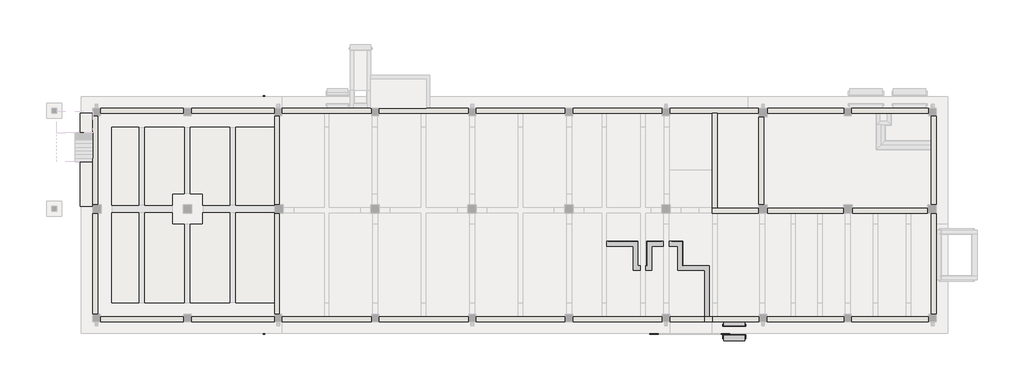
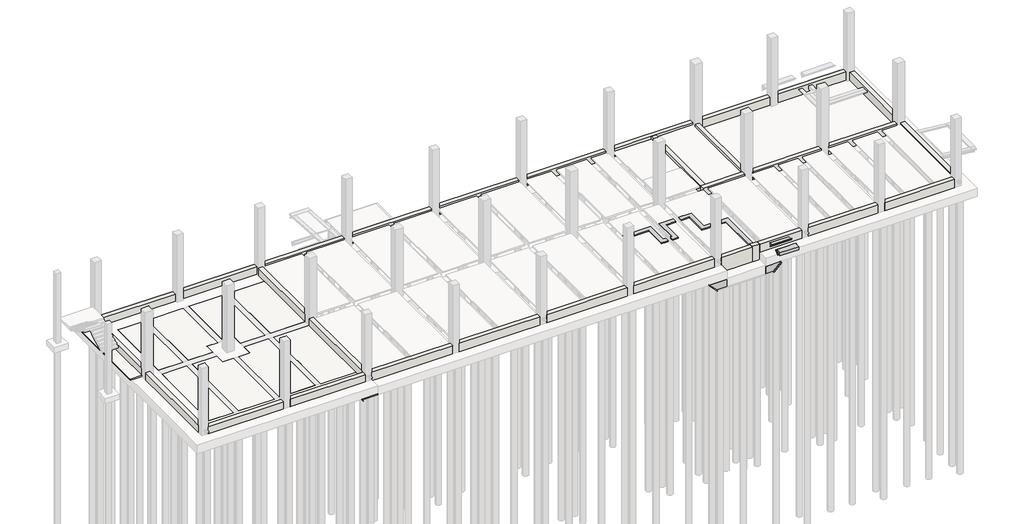
# One storey, part 1 of 7: 31 walls, 12 proxies, 4 slabs.
"""IFC4 building model written with IfcOpenShell, lengths in millimetres."""

from ifc_helpers import new_model, si_unit, frame, origin, place, context, project, spatial, polyline, outline, extrude, faceted_brep, element, save

model = new_model("IFC4")

# Units and contexts
model_context = context("Model", 3, world=origin())
ifc_project = project(units=[si_unit("LENGTHUNIT", "METRE", prefix="MILLI")], contexts=[model_context])

# Site, building, storey
site = spatial("IfcSite", under=ifc_project)
building = spatial("IfcBuilding", under=site)
storey = spatial("IfcBuildingStorey", under=building, Name="H.P.P", Elevation=4500.0)

# Proxies
placement = place(None, origin())
element("IfcBuildingElementProxy", 1, Name="H_SF_AR_S17_SOG Edge_1625x700", ObjectType="H_SF_AR_S17_SOG Edge_1625x700", at=placement, inside=storey, context=model_context, shape_type="SweptSolid", body=[
    extrude(outline(polyline([(2500.0, 47300.0), (3200.0, 47300.0), (3200.0, 45675.0), (2500.0, 46375.0), (2500.0, 47300.0)])), frame((0.0, -18250.0000001, 0.0), z_axis=(0.0, 1.0, 0.0), x_axis=(0.0, 0.0, 1.0)), (0.0, 0.0, 1.0), 2500.0),
])
element("IfcBuildingElementProxy", 2, Name="H_SF_AR_S17_SOG Edge_1400x700", ObjectType="H_SF_AR_S17_SOG Edge_1400x700", at=placement, inside=storey, context=model_context, shape_type="SweptSolid", body=[
    extrude(outline(polyline([(2500.0, 50825.0), (2500.0, 51525.0), (3200.0, 52225.0), (3200.0, 50825.0), (2500.0, 50825.0)])), frame((0.0, -18250.0000001, 0.0), z_axis=(0.0, 1.0, 0.0), x_axis=(0.0, 0.0, 1.0)), (0.0, 0.0, 1.0), 2500.0),
])
element("IfcBuildingElementProxy", 3, Name="H_SF_AR_S17_SOG Edge_1500x100", ObjectType="H_SF_AR_S17_SOG Edge_1500x100", at=placement, inside=storey, context=model_context, shape_type="SweptSolid", body=[
    extrude(outline(polyline([(3200.0, 15299.9999999), (3300.0, 15299.9999999), (3300.0, 13799.9999999), (3200.0, 13899.9999999), (3200.0, 15299.9999999)])), frame((0.0, -18250.0000001, 0.0), z_axis=(0.0, 1.0, 0.0), x_axis=(0.0, 0.0, 1.0)), (0.0, 0.0, 1.0), 2500.0),
    extrude(outline(polyline([(3200.0, 15299.9999999), (3300.0, 15299.9999999), (3300.0, 13799.9999999), (3200.0, 13899.9999999), (3200.0, 15299.9999999)])), frame((0.0, -1250.0000001, 0.0), z_axis=(0.0, 1.0, 0.0), x_axis=(0.0, 0.0, 1.0)), (0.0, 0.0, 1.0), 2500.0),
])
element("IfcBuildingElementProxy", 4, Name="H_SF_AR_S18_Lean_T50", ObjectType="H_SF_AR_S18_Lean_T50", at=placement, inside=storey, context=model_context, shape_type="SweptSolid", body=[
    extrude(outline(polyline([(3200.0, 52225.0), (2500.0, 51525.0), (2450.0, 51525.0), (2450.0, 51545.7106781), (3150.0, 52245.7106781), (3150.0, 52225.0), (3200.0, 52225.0)])), frame((0.0, -18350.0000001, 0.0), z_axis=(0.0, 1.0, 0.0), x_axis=(0.0, 0.0, 1.0)), (0.0, 0.0, 1.0), 2700.0),
])
element("IfcBuildingElementProxy", 5, Name="H_SF_AR_S18_Lean_T50", ObjectType="H_SF_AR_S18_Lean_T50", at=placement, inside=storey, context=model_context, shape_type="SweptSolid", body=[
    extrude(outline(polyline([(3200.0, 45675.0), (3150.0, 45675.0), (3150.0, 45654.2893219), (2450.0, 46354.2893219), (2450.0, 46375.0), (2500.0, 46375.0), (3200.0, 45675.0)])), frame((0.0, -18350.0000001, 0.0), z_axis=(0.0, 1.0, 0.0), x_axis=(0.0, 0.0, 1.0)), (0.0, 0.0, 1.0), 2700.0),
])
element("IfcBuildingElementProxy", 6, Name="H_SF_AR_S18_Lean_T50_100X100", ObjectType="H_SF_AR_S18_Lean_T50_100X100", at=placement, inside=storey, context=model_context, shape_type="SweptSolid", body=[
    extrude(outline(polyline([(3300.0, 13799.9999999), (3250.0, 13799.9999999), (3250.0, 13779.2893218), (3150.0, 13879.2893218), (3150.0, 13899.9999999), (3200.0, 13899.9999999), (3300.0, 13799.9999999)])), frame((0.0, -18350.0000001, 0.0), z_axis=(0.0, 1.0, 0.0), x_axis=(0.0, 0.0, 1.0)), (0.0, 0.0, 1.0), 2810.0),
    extrude(outline(polyline([(3300.0, 13799.9999999), (3250.0, 13799.9999999), (3250.0, 13779.2893218), (3150.0, 13879.2893218), (3150.0, 13899.9999999), (3200.0, 13899.9999999), (3300.0, 13799.9999999)])), frame((0.0, -1460.0000001, 0.0), z_axis=(0.0, 1.0, 0.0), x_axis=(0.0, 0.0, 1.0)), (0.0, 0.0, 1.0), 2810.0),
])
element("IfcBuildingElementProxy", 7, Name="H_SF_AR_B08_Stoop_T150_FrontEdge", ObjectType="H_SF_AR_B08_Stoop_T150_FrontEdge", at=placement, inside=storey, context=model_context, shape_type="SweptSolid", body=[
    extrude(outline(polyline([(-17312.0, 4450.0), (-17512.0, 4450.0), (-17662.0, 4600.0), (-17312.0, 4600.0), (-17312.0, 4450.0)])), frame((51775.0, 0.0, 0.0), z_axis=(1.0, 0.0, 0.0), x_axis=(0.0, 1.0, 0.0)), (0.0, 0.0, 1.0), 1700.0),
])
element("IfcBuildingElementProxy", 8, Name="H_SF_AR_B08_Stoop_T150_FrontEdge_500x300", ObjectType="H_SF_AR_B08_Stoop_T150_FrontEdge_500x300", at=placement, inside=storey, context=model_context, shape_type="Brep", body=[
    faceted_brep([(51775.0, -18899.9999926, 4300.0), (51775.0, -18899.9999926, 4600.0), (51775.0, -18599.9999926, 4600.0), (51775.0, -18399.9999926, 4600.0), (51775.0, -18699.9999926, 4300.0), (53475.0, -18899.9999926, 4300.0), (53475.0, -18699.9999926, 4300.0), (53475.0, -18399.9999926, 4600.0), (53475.0, -18599.9999926, 4600.0), (53475.0, -18899.9999926, 4600.0)], [[[0, 1, 2, 3, 4]], [[5, 6, 7, 8, 9]], [[1, 0, 5, 9]], [[3, 2, 1, 9, 8, 7]], [[4, 3, 7, 6]], [[0, 4, 6, 5]]]),
])
element("IfcBuildingElementProxy", 9, Name="H_SF_AR_S18_Lean_T50_300X300", ObjectType="H_SF_AR_S18_Lean_T50_300X300", at=placement, inside=storey, context=model_context, shape_type="SweptSolid", body=[
    extrude(outline(polyline([(-18699.9999926, 4250.0), (-18699.9999926, 4300.0), (-18399.9999926, 4600.0), (-18399.9999926, 4550.0), (-18379.2893145, 4550.0), (-18679.2893145, 4250.0), (-18699.9999926, 4250.0)])), frame((51675.0, 0.0, 0.0), z_axis=(1.0, 0.0, 0.0), x_axis=(0.0, 1.0, 0.0)), (0.0, 0.0, 1.0), 1900.0),
])
element("IfcBuildingElementProxy", 10, Name="H_SF_AR_S18_Lean_T50_150X150", ObjectType="H_SF_AR_S18_Lean_T50_150X150", at=placement, inside=storey, context=model_context, shape_type="SweptSolid", body=[
    extrude(outline(polyline([(-17512.0, 4450.0), (-17512.0, 4400.0), (-17532.7106781, 4400.0), (-17682.7106781, 4550.0), (-17662.0, 4550.0), (-17662.0, 4600.0), (-17512.0, 4450.0)])), frame((51675.0, 0.0, 0.0), z_axis=(1.0, 0.0, 0.0), x_axis=(0.0, 1.0, 0.0)), (0.0, 0.0, 1.0), 1900.0),
])
element("IfcBuildingElementProxy", 11, Name="H_SF_AR_S17_SOG Edge_450x150", ObjectType="H_SF_AR_S17_SOG Edge_450x150", at=placement, inside=storey, context=model_context, shape_type="Brep", body=[
    faceted_brep([(50175.0, -16900.0, 4550.0), (50475.0, -16900.0, 4550.0), (50575.0, -16900.0, 4650.0), (50175.0, -16900.0, 4650.0), (50175.0, -13075.0, 4550.0), (50175.0, -13075.0, 4650.0), (50475.0, -12775.0, 4550.0), (50575.0, -12675.0, 4650.0), (48375.0, -12675.0, 4650.0), (48375.0, -10675.0, 4650.0), (47250.0, -10675.0, 4650.0), (47250.0, -11075.0, 4650.0), (47975.0, -11075.0, 4650.0), (47975.0, -13075.0, 4650.0), (47975.0, -13075.0, 4550.0), (48275.0, -12775.0, 4550.0), (47975.0, -11075.0, 4550.0), (48275.0, -10775.0, 4550.0), (47250.0, -10775.0, 4550.0), (47250.0, -11075.0, 4550.0)], [[[0, 1, 2, 3]], [[4, 0, 3, 5]], [[1, 6, 7, 2]], [[4, 6, 1, 0]], [[3, 2, 7, 8, 9, 10, 11, 12, 13, 5]], [[4, 5, 13, 14]], [[7, 6, 15, 8]], [[6, 4, 14, 15]], [[14, 13, 12, 16]], [[8, 15, 17, 9]], [[15, 14, 16, 17]], [[18, 19, 11, 10]], [[16, 12, 11, 19]], [[9, 17, 18, 10]], [[17, 16, 19, 18]]]),
    faceted_brep([(46750.0, -11075.0, 4650.0), (46750.0, -10675.0, 4650.0), (45425.0, -10675.0, 4650.0), (45425.0, -12675.0, 4650.0), (45325.0, -12675.0, 4650.0), (45325.0, -13075.0, 4650.0), (45825.0, -13075.0, 4650.0), (45825.0, -11075.0, 4650.0), (46750.0, -11075.0, 4550.0), (46750.0, -10775.0, 4550.0), (45825.0, -11075.0, 4550.0), (45525.0, -10775.0, 4550.0), (45825.0, -13075.0, 4550.0), (45525.0, -12775.0, 4550.0), (45325.0, -12775.0, 4550.0), (45325.0, -13075.0, 4550.0)], [[[0, 1, 2, 3, 4, 5, 6, 7]], [[8, 9, 1, 0]], [[10, 8, 0, 7]], [[9, 11, 2, 1]], [[10, 11, 9, 8]], [[10, 7, 6, 12]], [[2, 11, 13, 3]], [[11, 10, 12, 13]], [[14, 15, 5, 4]], [[12, 6, 5, 15]], [[3, 13, 14, 4]], [[13, 12, 15, 14]]]),
    faceted_brep([(44875.0, -13075.0, 4650.0), (44875.0, -12675.0, 4650.0), (44675.0, -12675.0, 4650.0), (44675.0, -10675.0, 4650.0), (42125.0, -10675.0, 4650.0), (42125.0, -11075.0, 4650.0), (44275.0, -11075.0, 4650.0), (44275.0, -13075.0, 4650.0), (44875.0, -13075.0, 4550.0), (44875.0, -12775.0, 4550.0), (44275.0, -13075.0, 4550.0), (44575.0, -12775.0, 4550.0), (44275.0, -11075.0, 4550.0), (44575.0, -10775.0, 4550.0), (42125.0, -10775.0, 4550.0), (42125.0, -11075.0, 4550.0)], [[[0, 1, 2, 3, 4, 5, 6, 7]], [[8, 9, 1, 0]], [[10, 8, 0, 7]], [[9, 11, 2, 1]], [[10, 11, 9, 8]], [[10, 7, 6, 12]], [[2, 11, 13, 3]], [[11, 10, 12, 13]], [[14, 15, 5, 4]], [[12, 6, 5, 15]], [[3, 13, 14, 4]], [[13, 12, 15, 14]]]),
])
element("IfcBuildingElementProxy", 12, Name="H_SF_AR_S18_Lean_T50_100X100", ObjectType="H_SF_AR_S18_Lean_T50_100X100", at=placement, inside=storey, context=model_context, shape_type="Brep", body=[
    faceted_brep([(50575.0, -16790.0, 4540.0), (50475.0, -16790.0, 4440.0), (50475.0, -16790.0, 4390.0), (50495.7106781, -16790.0, 4390.0), (50595.7106781, -16790.0, 4490.0), (50575.0, -16790.0, 4490.0), (50575.0, -12675.0, 4490.0), (50575.0, -12675.0, 4540.0), (50595.7106781, -12654.2893219, 4490.0), (50495.7106781, -12754.2893219, 4390.0), (50475.0, -12775.0, 4390.0), (50475.0, -12775.0, 4440.0), (48375.0, -12675.0, 4540.0), (48275.0, -12775.0, 4440.0), (48275.0, -12775.0, 4390.0), (48295.7106781, -12754.2893219, 4390.0), (48395.7106781, -12654.2893219, 4490.0), (48375.0, -12675.0, 4490.0), (48375.0, -10675.0, 4540.0), (48275.0, -10775.0, 4440.0), (48275.0, -10775.0, 4390.0), (48295.7106781, -10754.2893219, 4390.0), (48395.7106781, -10654.2893219, 4490.0), (48375.0, -10675.0, 4490.0), (47360.0, -10675.0, 4540.0), (47360.0, -10675.0, 4490.0), (47360.0, -10654.2893219, 4490.0), (47360.0, -10754.2893219, 4390.0), (47360.0, -10775.0, 4390.0), (47360.0, -10775.0, 4440.0)], [[[0, 1, 2, 3, 4, 5]], [[0, 5, 6, 7]], [[5, 4, 8, 6]], [[4, 3, 9, 8]], [[3, 2, 10, 9]], [[2, 1, 11, 10]], [[1, 0, 7, 11]], [[11, 7, 12, 13]], [[10, 11, 13, 14]], [[9, 10, 14, 15]], [[8, 9, 15, 16]], [[6, 8, 16, 17]], [[7, 6, 17, 12]], [[13, 12, 18, 19]], [[14, 13, 19, 20]], [[15, 14, 20, 21]], [[16, 15, 21, 22]], [[17, 16, 22, 23]], [[12, 17, 23, 18]], [[24, 25, 26, 27, 28, 29]], [[19, 18, 24, 29]], [[20, 19, 29, 28]], [[21, 20, 28, 27]], [[22, 21, 27, 26]], [[23, 22, 26, 25]], [[18, 23, 25, 24]]]),
    faceted_brep([(46640.0, -10675.0, 4540.0), (46640.0, -10775.0, 4440.0), (46640.0, -10775.0, 4390.0), (46640.0, -10754.2893219, 4390.0), (46640.0, -10654.2893219, 4490.0), (46640.0, -10675.0, 4490.0), (45425.0, -10675.0, 4540.0), (45525.0, -10775.0, 4440.0), (45525.0, -10775.0, 4390.0), (45504.2893219, -10754.2893219, 4390.0), (45404.2893219, -10654.2893219, 4490.0), (45425.0, -10675.0, 4490.0), (45435.0, -10675.0, 4490.0), (45425.0, -12775.0, 4540.0), (45425.0, -12775.0, 4490.0), (45404.2893219, -12775.0, 4490.0), (45504.2893219, -12775.0, 4390.0), (45525.0, -12775.0, 4390.0), (45525.0, -12775.0, 4440.0)], [[[0, 1, 2, 3, 4, 5]], [[1, 0, 6, 7]], [[2, 1, 7, 8]], [[3, 2, 8, 9]], [[4, 3, 9, 10]], [[5, 4, 10, 11, 12]], [[0, 5, 12, 11, 6]], [[13, 14, 15, 16, 17, 18]], [[7, 6, 13, 18]], [[8, 7, 18, 17]], [[9, 8, 17, 16]], [[10, 9, 16, 15]], [[11, 10, 15, 14]], [[6, 11, 14, 13]]]),
    faceted_brep([(42235.0, -10675.0, 4540.0), (42235.0, -10675.0, 4490.0), (42235.0, -10654.2893219, 4490.0), (42235.0, -10754.2893219, 4390.0), (42235.0, -10775.0, 4390.0), (42235.0, -10775.0, 4440.0), (44575.0, -10775.0, 4440.0), (44675.0, -10675.0, 4540.0), (44575.0, -10775.0, 4390.0), (44595.7106781, -10754.2893219, 4390.0), (44695.7106781, -10654.2893219, 4490.0), (44675.0, -10675.0, 4490.0), (44575.0, -12775.0, 4440.0), (44675.0, -12675.0, 4540.0), (44575.0, -12775.0, 4390.0), (44595.7106781, -12754.2893219, 4390.0), (44695.7106781, -12654.2893219, 4490.0), (44675.0, -12675.0, 4490.0), (44765.0, -12675.0, 4540.0), (44765.0, -12775.0, 4440.0), (44765.0, -12775.0, 4390.0), (44765.0, -12754.2893219, 4390.0), (44765.0, -12654.2893219, 4490.0), (44765.0, -12675.0, 4490.0)], [[[0, 1, 2, 3, 4, 5]], [[6, 7, 0, 5]], [[8, 6, 5, 4]], [[9, 8, 4, 3]], [[10, 9, 3, 2]], [[11, 10, 2, 1]], [[7, 11, 1, 0]], [[12, 13, 7, 6]], [[14, 12, 6, 8]], [[15, 14, 8, 9]], [[16, 15, 9, 10]], [[17, 16, 10, 11]], [[13, 17, 11, 7]], [[18, 19, 20, 21, 22, 23]], [[19, 18, 13, 12]], [[20, 19, 12, 14]], [[21, 20, 14, 15]], [[22, 21, 15, 16]], [[23, 22, 16, 17]], [[18, 23, 17, 13]]]),
])

# Slabs
element("IfcSlab", 13, ObjectType="H_FL_AR_S17_RC Slab_T150_B1S1", at=placement, inside=storey, context=model_context, shape_type="Brep", body=[
    faceted_brep([(3500.0, -1250.0000001, 3950.0), (3500.0, -7700.0, 3950.0), (1250.0000002, -7700.0, 3950.0), (1250.0000002, -1250.0000001, 3950.0), (3500.0, -7700.0, 4100.0), (3500.0, -1250.0000001, 4100.0), (1250.0000002, -1250.0000001, 4100.0), (1250.0000002, -7700.0, 4100.0)], [[[0, 1, 2, 3]], [[4, 5, 6, 7]], [[1, 0, 5, 4]], [[2, 1, 4, 7]], [[3, 2, 7, 6]], [[0, 3, 6, 5]]]),
    faceted_brep([(1250.0000002, -8300.0, 3950.0), (3500.0, -8300.0, 3950.0), (3500.0, -15750.0000001, 3950.0), (1250.0000002, -15750.0000001, 3950.0), (3500.0, -8300.0, 4100.0), (1250.0000002, -8300.0, 4100.0), (1250.0000002, -15750.0000001, 4100.0), (3500.0, -15750.0000001, 4100.0)], [[[0, 1, 2, 3]], [[4, 5, 6, 7]], [[1, 0, 5, 4]], [[2, 1, 4, 7]], [[3, 2, 7, 6]], [[0, 3, 6, 5]]]),
    faceted_brep([(6250.0, -7700.0, 3950.0), (4000.0, -7700.0, 3950.0), (4000.0, -1250.0000001, 3950.0), (7250.0, -1250.0000001, 3950.0), (7250.0, -6750.0, 3950.0), (6250.0, -6750.0, 3950.0), (4000.0, -7700.0, 4100.0), (6250.0, -7700.0, 4100.0), (6250.0, -6750.0, 4100.0), (7250.0, -6750.0, 4100.0), (7250.0, -1250.0000001, 4100.0), (4000.0, -1250.0000001, 4100.0)], [[[0, 1, 2, 3, 4, 5]], [[6, 7, 8, 9, 10, 11]], [[1, 0, 7, 6]], [[2, 1, 6, 11]], [[3, 2, 11, 10]], [[4, 3, 10, 9]], [[5, 4, 9, 8]], [[0, 5, 8, 7]]]),
    faceted_brep([(6250.0, -8300.0, 3950.0), (6250.0, -9250.0, 3950.0), (7250.0, -9250.0, 3950.0), (7250.0, -15750.0000001, 3950.0), (4000.0, -15750.0000001, 3950.0), (4000.0, -8300.0, 3950.0), (6250.0, -9250.0, 4100.0), (6250.0, -8300.0, 4100.0), (4000.0, -8300.0, 4100.0), (4000.0, -15750.0000001, 4100.0), (7250.0, -15750.0000001, 4100.0), (7250.0, -9250.0, 4100.0)], [[[0, 1, 2, 3, 4, 5]], [[6, 7, 8, 9, 10, 11]], [[1, 0, 7, 6]], [[2, 1, 6, 11]], [[3, 2, 11, 10]], [[4, 3, 10, 9]], [[5, 4, 9, 8]], [[0, 5, 8, 7]]]),
    faceted_brep([(8750.0, -7700.0, 3950.0), (8750.0, -6750.0, 3950.0), (7750.0, -6750.0, 3950.0), (7750.0, -1250.0000001, 3950.0), (11000.0, -1250.0000001, 3950.0), (11000.0, -7700.0, 3950.0), (8750.0, -6750.0, 4100.0), (8750.0, -7700.0, 4100.0), (11000.0, -7700.0, 4100.0), (11000.0, -1250.0000001, 4100.0), (7750.0, -1250.0000001, 4100.0), (7750.0, -6750.0, 4100.0)], [[[0, 1, 2, 3, 4, 5]], [[6, 7, 8, 9, 10, 11]], [[1, 0, 7, 6]], [[2, 1, 6, 11]], [[3, 2, 11, 10]], [[4, 3, 10, 9]], [[5, 4, 9, 8]], [[0, 5, 8, 7]]]),
    faceted_brep([(8750.0, -8300.0, 3950.0), (11000.0, -8300.0, 3950.0), (11000.0, -15750.0000001, 3950.0), (7750.0, -15750.0000001, 3950.0), (7750.0, -9250.0, 3950.0), (8750.0, -9250.0, 3950.0), (11000.0, -8300.0, 4100.0), (8750.0, -8300.0, 4100.0), (8750.0, -9250.0, 4100.0), (7750.0, -9250.0, 4100.0), (7750.0, -15750.0000001, 4100.0), (11000.0, -15750.0000001, 4100.0)], [[[0, 1, 2, 3, 4, 5]], [[6, 7, 8, 9, 10, 11]], [[1, 0, 7, 6]], [[2, 1, 6, 11]], [[3, 2, 11, 10]], [[4, 3, 10, 9]], [[5, 4, 9, 8]], [[0, 5, 8, 7]]]),
    faceted_brep([(11500.0, -7699.9999999, 3950.0), (11500.0, -1250.0000001, 3950.0), (14700.0000001, -1250.0000001, 3950.0), (14700.0000001, -6750.0, 3950.0), (13800.0000001, -6750.0, 3950.0), (13800.0000001, -7699.9999999, 3950.0), (14700.0000001, -7699.9999999, 4100.0), (14700.0000001, -7650.0, 4100.0), (14700.0000001, -1250.0000001, 4100.0), (11500.0, -1250.0000001, 4100.0), (11500.0, -7699.9999999, 4100.0), (14700.0000001, -7699.9999999, 4000.0), (14700.0000001, -7650.0, 4000.0), (14700.0000001, -6750.0, 4000.0), (13800.0000001, -7699.9999999, 4000.0), (13800.0000001, -6750.0, 4000.0)], [[[0, 1, 2, 3, 4, 5]], [[6, 7, 8, 9, 10]], [[8, 7, 6, 11, 12, 13, 3, 2]], [[6, 10, 0, 5, 14, 11]], [[1, 0, 10, 9]], [[2, 1, 9, 8]], [[14, 15, 13, 12, 11]], [[13, 15, 4, 3]], [[15, 14, 5, 4]]]),
    faceted_brep([(14700.0, -15750.0000001, 3950.0), (11500.0, -15750.0000001, 3950.0), (11500.0, -8299.9999999, 3950.0), (13800.0000001, -8299.9999999, 3950.0), (13800.0000001, -9250.0, 3950.0), (14700.0, -9250.0, 3950.0), (14700.0, -15750.0000001, 4100.0), (14700.0, -8350.0, 4100.0), (14700.0, -8299.9999999, 4100.0), (11500.0, -8299.9999999, 4100.0), (11500.0, -15750.0000001, 4100.0), (14700.0, -9250.0, 4000.0), (14700.0, -8350.0, 4000.0), (14700.0, -8299.9999999, 4000.0), (13800.0000001, -8299.9999999, 4000.0), (13800.0000001, -9250.0, 4000.0)], [[[0, 1, 2, 3, 4, 5]], [[6, 7, 8, 9, 10]], [[8, 7, 6, 0, 5, 11, 12, 13]], [[1, 0, 6, 10]], [[2, 1, 10, 9]], [[9, 8, 13, 14, 3, 2]], [[11, 15, 14, 13, 12]], [[14, 15, 4, 3]], [[15, 11, 5, 4]]]),
])
element("IfcSlab", 14, ObjectType="H_FL_AR_B07_Ground Insulation_T110", at=placement, inside=storey, context=model_context, shape_type="SweptSolid", body=[
    extrude(outline(polyline([(3500.0, -1250.0000001), (3500.0, -7700.0), (1250.0000002, -7700.0), (1250.0000002, -1250.0000001), (3500.0, -1250.0000001)])), frame((0.0, 0.0, 3840.0), z_axis=(0.0, 0.0, 1.0), x_axis=(1.0, 0.0, 0.0)), (0.0, 0.0, 1.0), 110.0),
    extrude(outline(polyline([(3500.0, -8300.0), (3500.0, -15750.0000001), (1250.0000002, -15750.0000001), (1250.0000002, -8300.0), (3500.0, -8300.0)])), frame((0.0, 0.0, 3840.0), z_axis=(0.0, 0.0, 1.0), x_axis=(1.0, 0.0, 0.0)), (0.0, 0.0, 1.0), 110.0),
    extrude(outline(polyline([(6250.0, -8300.0), (6250.0, -9250.0), (7250.0, -9250.0), (7250.0, -15750.0000001), (4000.0, -15750.0000001), (4000.0, -8300.0), (6250.0, -8300.0)])), frame((0.0, 0.0, 3840.0), z_axis=(0.0, 0.0, 1.0), x_axis=(1.0, 0.0, 0.0)), (0.0, 0.0, 1.0), 110.0),
    extrude(outline(polyline([(6250.0, -7700.0), (4000.0, -7700.0), (4000.0, -1250.0000001), (7250.0, -1250.0000001), (7250.0, -6750.0), (6250.0, -6750.0), (6250.0, -7700.0)])), frame((0.0, 0.0, 3840.0), z_axis=(0.0, 0.0, 1.0), x_axis=(1.0, 0.0, 0.0)), (0.0, 0.0, 1.0), 110.0),
    extrude(outline(polyline([(8750.0, -8300.0), (11000.0, -8300.0), (11000.0, -15750.0000001), (7750.0, -15750.0000001), (7750.0, -9250.0), (8750.0, -9250.0), (8750.0, -8300.0)])), frame((0.0, 0.0, 3840.0), z_axis=(0.0, 0.0, 1.0), x_axis=(1.0, 0.0, 0.0)), (0.0, 0.0, 1.0), 110.0),
    extrude(outline(polyline([(8750.0, -7700.0), (8750.0, -6750.0), (7750.0, -6750.0), (7750.0, -1250.0000001), (11000.0, -1250.0000001), (11000.0, -7700.0), (8750.0, -7700.0)])), frame((0.0, 0.0, 3840.0), z_axis=(0.0, 0.0, 1.0), x_axis=(1.0, 0.0, 0.0)), (0.0, 0.0, 1.0), 110.0),
    extrude(outline(polyline([(13800.0000001, -8300.0), (13800.0000001, -9250.0), (14700.0, -9250.0), (14700.0, -15750.0000001), (11500.0, -15750.0000001), (11500.0, -8300.0), (13800.0000001, -8300.0)])), frame((0.0, 0.0, 3840.0), z_axis=(0.0, 0.0, 1.0), x_axis=(1.0, 0.0, 0.0)), (0.0, 0.0, 1.0), 110.0),
    extrude(outline(polyline([(13800.0000001, -7700.0), (11500.0, -7700.0), (11500.0, -1250.0000001), (14700.0, -1250.0000001), (14700.0, -6750.0), (13800.0000001, -6750.0), (13800.0000001, -7700.0)])), frame((0.0, 0.0, 3840.0), z_axis=(0.0, 0.0, 1.0), x_axis=(1.0, 0.0, 0.0)), (0.0, 0.0, 1.0), 110.0),
])
element("IfcSlab", 15, ObjectType="H_FL_AR_B07_Ground Insulation_T110", at=placement, inside=storey, context=model_context, shape_type="Brep", body=[
    faceted_brep([(50575.0, -16900.0, 4540.0), (50575.0, -16900.0, 4650.0), (50475.0, -16900.0, 4550.0), (50475.0, -16900.0, 4440.0), (50475.0, -12775.0, 4550.0), (50475.0, -12775.0, 4440.0), (48275.0, -12775.0, 4550.0), (48275.0, -12775.0, 4440.0), (48375.0, -12675.0, 4540.0), (48375.0, -12675.0, 4650.0), (50575.0, -12675.0, 4650.0), (50575.0, -12675.0, 4540.0), (47459.9999996, -10675.0, 4540.0), (47459.9999996, -10675.0, 4650.0), (48375.0, -10675.0, 4650.0), (48375.0, -10675.0, 4540.0), (48275.0, -10775.0, 4440.0), (48275.0, -10775.0, 4550.0), (47459.9999996, -10775.0, 4550.0), (47459.9999996, -10775.0, 4440.0)], [[[0, 1, 2, 3]], [[3, 2, 4, 5]], [[5, 4, 6, 7]], [[8, 9, 10, 11]], [[11, 10, 1, 0]], [[10, 4, 2, 1]], [[11, 0, 3, 5]], [[12, 13, 14, 15]], [[16, 17, 18, 19]], [[19, 18, 13, 12]], [[7, 6, 17, 16]], [[15, 14, 9, 8]], [[18, 17, 14, 13]], [[10, 9, 6, 4]], [[19, 12, 15, 16]], [[11, 5, 7, 8]], [[9, 14, 17, 6]], [[8, 7, 16, 15]]]),
    faceted_brep([(46640.0, -10675.0, 4540.0), (46640.0, -10675.0, 4650.0), (46640.0, -10775.0, 4550.0), (46640.0, -10775.0, 4440.0), (45525.0, -10775.0, 4550.0), (45525.0, -10775.0, 4440.0), (45525.0, -12775.0, 4550.0), (45525.0, -12775.0, 4440.0), (45325.0, -12775.0, 4550.0), (45325.0, -12775.0, 4440.0), (45425.0, -12675.0, 4540.0), (45425.0, -12675.0, 4650.0), (45425.0, -10675.0, 4650.0), (45425.0, -10675.0, 4540.0), (45325.0, -12675.0, 4650.0), (45325.0, -12675.0, 4540.0)], [[[0, 1, 2, 3]], [[3, 2, 4, 5]], [[5, 4, 6, 7]], [[7, 6, 8, 9]], [[10, 11, 12, 13]], [[13, 12, 1, 0]], [[12, 4, 2, 1]], [[13, 0, 3, 5]], [[9, 8, 14, 15]], [[15, 14, 11, 10]], [[6, 11, 14, 8]], [[12, 11, 6, 4]], [[7, 9, 15, 10]], [[13, 5, 7, 10]]]),
    faceted_brep([(42235.0, -10675.0, 4540.0), (42235.0, -10675.0, 4650.0), (44675.0, -10675.0, 4650.0), (44675.0, -10675.0, 4540.0), (44675.0, -12675.0, 4650.0), (44675.0, -12675.0, 4540.0), (44875.0, -12775.0, 4440.0), (44875.0, -12775.0, 4550.0), (44575.0, -12775.0, 4550.0), (44575.0, -12775.0, 4440.0), (44575.0, -10775.0, 4550.0), (44575.0, -10775.0, 4440.0), (42235.0, -10775.0, 4550.0), (42235.0, -10775.0, 4440.0), (44875.0, -12675.0, 4650.0), (44875.0, -12675.0, 4540.0)], [[[0, 1, 2, 3]], [[3, 2, 4, 5]], [[6, 7, 8, 9]], [[9, 8, 10, 11]], [[11, 10, 12, 13]], [[13, 12, 1, 0]], [[12, 10, 2, 1]], [[13, 0, 3, 11]], [[10, 8, 4, 2]], [[11, 3, 5, 9]], [[5, 4, 14, 15]], [[15, 14, 7, 6]], [[8, 7, 14, 4]], [[9, 5, 15, 6]]]),
])
element("IfcSlab", 16, ObjectType="H_FL_AR_B07_Ground Insulation_T110", at=placement, inside=storey, context=model_context, shape_type="SweptSolid", body=[
    extrude(outline(polyline([(-300.0, -100.0), (-300.0, -7800.0), (-1360.0, -7800.0), (-1360.0, -100.0), (-300.0, -100.0)])), frame((0.0, 0.0, 4100.0), z_axis=(0.0, 0.0, 1.0), x_axis=(1.0, 0.0, 0.0)), (0.0, 0.0, 1.0), 110.0),
])

# Walls
element("IfcWall", 17, ObjectType="H_WA_AR_B02_Ext Wall RC-UG_T400_W1A", at=placement, inside=storey, context=model_context, shape_type="Brep", body=[
    faceted_brep([(300.0, -17300.0, 4100.0), (7200.0, -17300.0, 4100.0), (7200.0, -17300.0, 4800.0), (300.0, -17300.0, 4800.0), (300.0, -16900.0, 4100.0), (300.0, -16900.0, 4800.0), (7200.0, -16900.0, 4800.0), (7200.0, -16900.0, 4100.0), (7200.0, -17050.0, 4800.0), (300.0, -17050.0, 4800.0)], [[[0, 1, 2, 3]], [[4, 5, 6, 7]], [[1, 0, 4, 7]], [[2, 1, 7, 6, 8]], [[3, 2, 8, 6, 5, 9]], [[0, 3, 9, 5, 4]]]),
])
element("IfcWall", 18, ObjectType="H_WA_AR_B02_Ext Wall RC-UG_T400_W1A", at=placement, inside=storey, context=model_context, shape_type="Brep", body=[
    faceted_brep([(7800.0, -17300.0, 4100.0), (14700.0, -17300.0, 4100.0), (14700.0, -17300.0, 4800.0), (7800.0, -17300.0, 4800.0), (7800.0, -16900.0, 4100.0), (7800.0, -16900.0, 4800.0), (14700.0, -16900.0, 4800.0), (14700.0, -16900.0, 4100.0), (14700.0, -17050.0, 4800.0), (7800.0, -17050.0, 4800.0)], [[[0, 1, 2, 3]], [[4, 5, 6, 7]], [[1, 0, 4, 7]], [[2, 1, 7, 6, 8]], [[3, 2, 8, 6, 5, 9]], [[0, 3, 9, 5, 4]]]),
])
element("IfcWall", 19, ObjectType="H_WA_AR_B02_Ext Wall RC-UG_T400_W1A", at=placement, inside=storey, context=model_context, shape_type="Brep", body=[
    faceted_brep([(15299.9999999, -17300.0, 4000.0), (22700.0, -17300.0, 4000.0), (22700.0, -17300.0, 4800.0), (15299.9999999, -17300.0, 4800.0), (15299.9999999, -17300.0, 4100.0), (15299.9999999, -16900.0, 4000.0), (15299.9999999, -16900.0, 4800.0), (22700.0, -16900.0, 4800.0), (22700.0, -16900.0, 4000.0), (22700.0, -17050.0, 4800.0), (15299.9999999, -17050.0, 4800.0)], [[[0, 1, 2, 3, 4]], [[5, 6, 7, 8]], [[1, 0, 5, 8]], [[2, 1, 8, 7, 9]], [[3, 2, 9, 7, 6, 10]], [[0, 4, 3, 10, 6, 5]]]),
])
element("IfcWall", 20, ObjectType="H_WA_AR_B02_Ext Wall RC-UG_T400_W1A", at=placement, inside=storey, context=model_context, shape_type="Brep", body=[
    faceted_brep([(23300.0, -17300.0, 4000.0), (30700.0, -17300.0, 4000.0), (30700.0, -17300.0, 4800.0), (23300.0, -17300.0, 4800.0), (23300.0, -16900.0, 4000.0), (23300.0, -16900.0, 4800.0), (30700.0, -16900.0, 4800.0), (30700.0, -16900.0, 4000.0), (30700.0, -17050.0, 4800.0), (23300.0, -17050.0, 4800.0)], [[[0, 1, 2, 3]], [[4, 5, 6, 7]], [[1, 0, 4, 7]], [[2, 1, 7, 6, 8]], [[3, 2, 8, 6, 5, 9]], [[0, 3, 9, 5, 4]]]),
])
element("IfcWall", 21, ObjectType="H_WA_AR_B02_Ext Wall RC-UG_T400_W1A", at=placement, inside=storey, context=model_context, shape_type="Brep", body=[
    faceted_brep([(31300.0, -17300.0, 4000.0), (38700.0, -17300.0, 4000.0), (38700.0, -17300.0, 4800.0), (31300.0, -17300.0, 4800.0), (31300.0, -16900.0, 4000.0), (31300.0, -16900.0, 4800.0), (38700.0, -16900.0, 4800.0), (38700.0, -16900.0, 4000.0), (38700.0, -17050.0, 4800.0), (31300.0, -17050.0, 4800.0)], [[[0, 1, 2, 3]], [[4, 5, 6, 7]], [[1, 0, 4, 7]], [[2, 1, 7, 6, 8]], [[3, 2, 8, 6, 5, 9]], [[0, 3, 9, 5, 4]]]),
])
element("IfcWall", 22, ObjectType="H_WA_AR_B02_Ext Wall RC-UG_T400_W1A", at=placement, inside=storey, context=model_context, shape_type="Brep", body=[
    faceted_brep([(39300.0, -17300.0, 4000.0), (46700.0, -17300.0, 4000.0), (46700.0, -17300.0, 4800.0), (39300.0, -17300.0, 4800.0), (39300.0, -16900.0, 4000.0), (39300.0, -16900.0, 4800.0), (46700.0, -16900.0, 4800.0), (46700.0, -16900.0, 4000.0), (46700.0, -17050.0, 4800.0), (39300.0, -17050.0, 4800.0)], [[[0, 1, 2, 3]], [[4, 5, 6, 7]], [[1, 0, 4, 7]], [[2, 1, 7, 6, 8]], [[3, 2, 8, 6, 5, 9]], [[0, 3, 9, 5, 4]]]),
])
element("IfcWall", 23, ObjectType="H_WA_AR_B02_Ext Wall RC-UG_T400_W1A", at=placement, inside=storey, context=model_context, shape_type="Brep", body=[
    faceted_brep([(47300.0, -17300.0, 3300.0), (50175.0, -17300.0, 3300.0), (50175.0, -17300.0, 4700.0), (47300.0, -17300.0, 4700.0), (47300.0, -17300.0, 4000.0), (47300.0, -16900.0, 3300.0), (47300.0, -16900.0, 4700.0), (50175.0, -16900.0, 4700.0), (50175.0, -16900.0, 3300.0), (50175.0, -17050.0, 4700.0), (47300.0, -17050.0, 4700.0)], [[[0, 1, 2, 3, 4]], [[5, 6, 7, 8]], [[1, 0, 5, 8]], [[2, 1, 8, 7, 9]], [[3, 2, 9, 7, 6, 10]], [[0, 4, 3, 10, 6, 5]]]),
])
element("IfcWall", 24, ObjectType="H_WA_AR_B02_Ext Wall RC-UG_T400_W1A", at=placement, inside=storey, context=model_context, shape_type="Brep", body=[
    faceted_brep([(50175.0, -17300.0, 3300.0), (50825.0, -17300.0, 3300.0), (50825.0, -17300.0, 4000.0), (50825.0, -17300.0, 4800.0), (50175.0, -17300.0, 4800.0), (50175.0, -17300.0, 4700.0), (50175.0, -16900.0, 3300.0), (50175.0, -16900.0, 4700.0), (50175.0, -16900.0, 4800.0), (50825.0, -16900.0, 4800.0), (50825.0, -16900.0, 4000.0), (50825.0, -16900.0, 3300.0), (50175.0, -17050.0, 4800.0)], [[[0, 1, 2, 3, 4, 5]], [[6, 7, 8, 9, 10, 11]], [[1, 0, 6, 11]], [[3, 2, 1, 11, 10, 9]], [[4, 3, 9, 8, 12]], [[0, 5, 4, 12, 8, 7, 6]]]),
])
element("IfcWall", 25, ObjectType="H_WA_AR_B02_Ext Wall RC-UG_T400_W1A", at=placement, inside=storey, context=model_context, shape_type="Brep", body=[
    faceted_brep([(50825.0, -17300.0, 4000.0), (54700.0, -17300.0, 4000.0), (54700.0, -17300.0, 4800.0), (53175.0, -17300.0, 4800.0), (52075.0, -17300.0, 4800.0), (50825.0, -17300.0, 4800.0), (50825.0, -16900.0, 4000.0), (50825.0, -16900.0, 4800.0), (54700.0, -16900.0, 4800.0), (54700.0, -16900.0, 4000.0), (54700.0, -17050.0, 4800.0)], [[[0, 1, 2, 3, 4, 5]], [[6, 7, 8, 9]], [[1, 0, 6, 9]], [[2, 1, 9, 8, 10]], [[5, 4, 3, 2, 10, 8, 7]], [[0, 5, 7, 6]]]),
])
element("IfcWall", 26, ObjectType="H_WA_AR_B02_Ext Wall RC-UG_T400_W1A", at=placement, inside=storey, context=model_context, shape_type="Brep", body=[
    faceted_brep([(55300.0, -17300.0, 4000.0), (61700.0, -17300.0, 4000.0), (61700.0, -17300.0, 4800.0), (55300.0, -17300.0, 4800.0), (55300.0, -16900.0, 4000.0), (55300.0, -16900.0, 4800.0), (61700.0, -16900.0, 4800.0), (61700.0, -16900.0, 4000.0), (61700.0, -17050.0, 4800.0), (55300.0, -17050.0, 4800.0)], [[[0, 1, 2, 3]], [[4, 5, 6, 7]], [[1, 0, 4, 7]], [[2, 1, 7, 6, 8]], [[3, 2, 8, 6, 5, 9]], [[0, 3, 9, 5, 4]]]),
])
element("IfcWall", 27, ObjectType="H_WA_AR_B02_Ext Wall RC-UG_T400_W1A", at=placement, inside=storey, context=model_context, shape_type="Brep", body=[
    faceted_brep([(62300.0, -17300.0, 4000.0), (68700.0, -17300.0, 4000.0), (68700.0, -17300.0, 4800.0), (62300.0, -17300.0, 4800.0), (62300.0, -16900.0, 4000.0), (62300.0, -16900.0, 4800.0), (68700.0, -16900.0, 4800.0), (68700.0, -16900.0, 4000.0), (68700.0, -17050.0, 4800.0), (62300.0, -17050.0, 4800.0)], [[[0, 1, 2, 3]], [[4, 5, 6, 7]], [[1, 0, 4, 7]], [[2, 1, 7, 6, 8]], [[3, 2, 8, 6, 5, 9]], [[0, 3, 9, 5, 4]]]),
])
element("IfcWall", 28, ObjectType="H_WA_AR_B02_Ext Wall RC-UG_T400_W1A", at=placement, inside=storey, context=model_context, shape_type="Brep", body=[
    faceted_brep([(69300.0, -16700.0, 4000.0), (69300.0, -8350.0, 4000.0), (69300.0, -8350.0, 4800.0), (69300.0, -10250.0, 4800.0), (69300.0, -13350.0, 4800.0), (69300.0, -16700.0, 4800.0), (68900.0, -16700.0, 4000.0), (68900.0, -16700.0, 4800.0), (68900.0, -8350.0, 4800.0), (68900.0, -8350.0, 4000.0), (69050.0, -8350.0, 4800.0), (69050.0, -16700.0, 4800.0)], [[[0, 1, 2, 3, 4, 5]], [[6, 7, 8, 9]], [[1, 0, 6, 9]], [[2, 1, 9, 8, 10]], [[5, 4, 3, 2, 10, 8, 7, 11]], [[0, 5, 11, 7, 6]]]),
])
element("IfcWall", 29, ObjectType="H_WA_AR_B02_Ext Wall RC-UG_T400_W1A", at=placement, inside=storey, context=model_context, shape_type="Brep", body=[
    faceted_brep([(69300.0, -7650.0, 4000.0), (69300.0, -300.0, 4000.0), (69300.0, -300.0, 4800.0), (69300.0, -7650.0, 4800.0), (68900.0, -7650.0, 4000.0), (68900.0, -7650.0, 4800.0), (68900.0, -300.0, 4800.0), (68900.0, -300.0, 4000.0), (69050.0, -300.0, 4800.0), (69050.0, -7650.0, 4800.0)], [[[0, 1, 2, 3]], [[4, 5, 6, 7]], [[1, 0, 4, 7]], [[2, 1, 7, 6, 8]], [[3, 2, 8, 6, 5, 9]], [[0, 3, 9, 5, 4]]]),
])
element("IfcWall", 30, ObjectType="H_WA_AR_B02_Ext Wall RC-UG_T400_W1A", at=placement, inside=storey, context=model_context, shape_type="Brep", body=[
    faceted_brep([(68700.0, 300.0, 4000.0), (62300.0, 300.0, 4000.0), (62300.0, 300.0, 4800.0), (62450.0, 300.0, 4800.0), (64550.0, 300.0, 4800.0), (66050.0, 300.0, 4800.0), (68150.0, 300.0, 4800.0), (68700.0, 300.0, 4800.0), (68700.0, -100.0, 4000.0), (68700.0, -100.0, 4800.0), (62300.0, -100.0, 4800.0), (62300.0, -100.0, 4000.0), (62300.0, 50.0, 4800.0), (68700.0, 50.0, 4800.0)], [[[0, 1, 2, 3, 4, 5, 6, 7]], [[8, 9, 10, 11]], [[1, 0, 8, 11]], [[2, 1, 11, 10, 12]], [[7, 6, 5, 4, 3, 2, 12, 10, 9, 13]], [[0, 7, 13, 9, 8]]]),
])
element("IfcWall", 31, ObjectType="H_WA_AR_B02_Ext Wall RC-UG_T400_W1A", at=placement, inside=storey, context=model_context, shape_type="Brep", body=[
    faceted_brep([(61700.0, 300.0, 4000.0), (55350.0, 300.0, 4000.0), (55350.0, 300.0, 4800.0), (61700.0, 300.0, 4800.0), (61700.0, -100.0, 4000.0), (61700.0, -100.0, 4800.0), (55350.0, -100.0, 4800.0), (55350.0, -100.0, 4000.0), (55350.0, 50.0, 4800.0), (61700.0, 50.0, 4800.0)], [[[0, 1, 2, 3]], [[4, 5, 6, 7]], [[1, 0, 4, 7]], [[2, 1, 7, 6, 8]], [[3, 2, 8, 6, 5, 9]], [[0, 3, 9, 5, 4]]]),
])
element("IfcWall", 32, ObjectType="H_WA_AR_B02_Ext Wall RC-UG_T400_W1A", at=placement, inside=storey, context=model_context, shape_type="Brep", body=[
    faceted_brep([(54650.0, 300.0, 4000.0), (47300.0, 300.0, 4000.0), (47300.0, 300.0, 4800.0), (54650.0, 300.0, 4800.0), (54650.0, -100.0, 4000.0), (54650.0, -100.0, 4800.0), (51225.0, -100.0, 4800.0), (50825.0, -100.0, 4800.0), (47300.0, -100.0, 4800.0), (47300.0, -100.0, 4000.0), (50825.0, -100.0, 4000.0), (51225.0, -100.0, 4000.0), (47300.0, 50.0, 4800.0), (54650.0, 50.0, 4800.0)], [[[0, 1, 2, 3]], [[4, 5, 6, 7, 8, 9, 10, 11]], [[1, 0, 4, 11, 10, 9]], [[2, 1, 9, 8, 12]], [[3, 2, 12, 8, 7, 6, 5, 13]], [[0, 3, 13, 5, 4]]]),
])
element("IfcWall", 33, ObjectType="H_WA_AR_B02_Ext Wall RC-UG_T400_W1A", at=placement, inside=storey, context=model_context, shape_type="Brep", body=[
    faceted_brep([(46700.0, 300.0, 4000.0), (39300.0, 300.0, 4000.0), (39300.0, 300.0, 4800.0), (46700.0, 300.0, 4800.0), (46700.0, -100.0, 4000.0), (46700.0, -100.0, 4800.0), (39300.0, -100.0, 4800.0), (39300.0, -100.0, 4000.0), (39300.0, 50.0, 4800.0), (46700.0, 50.0, 4800.0)], [[[0, 1, 2, 3]], [[4, 5, 6, 7]], [[1, 0, 4, 7]], [[2, 1, 7, 6, 8]], [[3, 2, 8, 6, 5, 9]], [[0, 3, 9, 5, 4]]]),
])
element("IfcWall", 34, ObjectType="H_WA_AR_B02_Ext Wall RC-UG_T400_W1A", at=placement, inside=storey, context=model_context, shape_type="Brep", body=[
    faceted_brep([(38700.0, 300.0, 4000.0), (31300.0, 300.0, 4000.0), (31300.0, 300.0, 4800.0), (38700.0, 300.0, 4800.0), (38700.0, -100.0, 4000.0), (38700.0, -100.0, 4800.0), (31300.0, -100.0, 4800.0), (31300.0, -100.0, 4000.0), (31300.0, 50.0, 4800.0), (38700.0, 50.0, 4800.0)], [[[0, 1, 2, 3]], [[4, 5, 6, 7]], [[1, 0, 4, 7]], [[2, 1, 7, 6, 8]], [[3, 2, 8, 6, 5, 9]], [[0, 3, 9, 5, 4]]]),
])
element("IfcWall", 35, ObjectType="H_WA_AR_B02_Ext Wall RC-UG_T400_W1A", at=placement, inside=storey, context=model_context, shape_type="Brep", body=[
    faceted_brep([(30700.0, 300.0, 4000.0), (23300.0, 300.0, 4000.0), (23300.0, 300.0, 4800.0), (30700.0, 300.0, 4800.0), (30700.0, -100.0, 4000.0), (30700.0, -100.0, 4800.0), (23300.0, -100.0, 4800.0), (23300.0, -100.0, 4000.0), (23300.0, 50.0, 4800.0), (30700.0, 50.0, 4800.0)], [[[0, 1, 2, 3]], [[4, 5, 6, 7]], [[1, 0, 4, 7]], [[2, 1, 7, 6, 8]], [[3, 2, 8, 6, 5, 9]], [[0, 3, 9, 5, 4]]]),
])
element("IfcWall", 36, ObjectType="H_WA_AR_B02_Ext Wall RC-UG_T400_W1A", at=placement, inside=storey, context=model_context, shape_type="Brep", body=[
    faceted_brep([(22700.0, 300.0, 4000.0), (15300.0, 300.0, 4000.0), (15300.0, 300.0, 4100.0), (15300.0, 300.0, 4800.0), (22690.0, 300.0, 4800.0), (22700.0, 300.0, 4800.0), (22700.0, -100.0, 4000.0), (22700.0, -100.0, 4800.0), (15300.0, -100.0, 4800.0), (15300.0, -100.0, 4000.0), (15300.0, 50.0, 4800.0)], [[[0, 1, 2, 3, 4, 5]], [[6, 7, 8, 9]], [[1, 0, 6, 9]], [[3, 2, 1, 9, 8, 10]], [[5, 4, 3, 10, 8, 7]], [[0, 5, 7, 6]]]),
])
element("IfcWall", 37, ObjectType="H_WA_AR_B02_Ext Wall RC-UG_T400_W1A", at=placement, inside=storey, context=model_context, shape_type="Brep", body=[
    faceted_brep([(14700.0, 300.0, 4100.0), (7800.0, 300.0, 4100.0), (7800.0, 300.0, 4800.0), (14700.0, 300.0, 4800.0), (14700.0, -100.0, 4100.0), (14700.0, -100.0, 4800.0), (7800.0, -100.0, 4800.0), (7800.0, -100.0, 4100.0), (7800.0, 50.0, 4800.0), (14700.0, 50.0, 4800.0)], [[[0, 1, 2, 3]], [[4, 5, 6, 7]], [[1, 0, 4, 7]], [[2, 1, 7, 6, 8]], [[3, 2, 8, 6, 5, 9]], [[0, 3, 9, 5, 4]]]),
])
element("IfcWall", 38, ObjectType="H_WA_AR_B02_Ext Wall RC-UG_T400_W1A", at=placement, inside=storey, context=model_context, shape_type="Brep", body=[
    faceted_brep([(7200.0, 300.0, 4100.0), (300.0, 300.0, 4100.0), (300.0, 300.0, 4800.0), (7200.0, 300.0, 4800.0), (7200.0, -100.0, 4100.0), (7200.0, -100.0, 4800.0), (300.0, -100.0, 4800.0), (300.0, -100.0, 4100.0), (300.0, 50.0, 4800.0), (7200.0, 50.0, 4800.0)], [[[0, 1, 2, 3]], [[4, 5, 6, 7]], [[1, 0, 4, 7]], [[2, 1, 7, 6, 8]], [[3, 2, 8, 6, 5, 9]], [[0, 3, 9, 5, 4]]]),
])
element("IfcWall", 39, ObjectType="H_WA_AR_B02_Ext Wall RC-UG_T400_W1A", at=placement, inside=storey, context=model_context, shape_type="Brep", body=[
    faceted_brep([(-300.0, -300.0, 4100.0), (-300.0, -7650.0, 4100.0), (-300.0, -7650.0, 4800.0), (-300.0, -300.0, 4800.0), (100.0, -300.0, 4100.0), (100.0, -300.0, 4800.0), (100.0, -7650.0, 4800.0), (100.0, -7650.0, 4100.0), (-50.0, -7650.0, 4800.0), (-50.0, -300.0, 4800.0)], [[[0, 1, 2, 3]], [[4, 5, 6, 7]], [[1, 0, 4, 7]], [[2, 1, 7, 6, 8]], [[3, 2, 8, 6, 5, 9]], [[0, 3, 9, 5, 4]]]),
])
element("IfcWall", 40, ObjectType="H_WA_AR_B02_Ext Wall RC-UG_T400_W1A", at=placement, inside=storey, context=model_context, shape_type="Brep", body=[
    faceted_brep([(-300.0, -8350.0, 4100.0), (-300.0, -16700.0, 4100.0), (-300.0, -16700.0, 4800.0), (-300.0, -8350.0, 4800.0), (100.0, -8350.0, 4100.0), (100.0, -8350.0, 4800.0), (100.0, -16700.0, 4800.0), (100.0, -16700.0, 4100.0), (-50.0, -16700.0, 4800.0), (-50.0, -8350.0, 4800.0)], [[[0, 1, 2, 3]], [[4, 5, 6, 7]], [[1, 0, 4, 7]], [[2, 1, 7, 6, 8]], [[3, 2, 8, 6, 5, 9]], [[0, 3, 9, 5, 4]]]),
])
element("IfcWall", 41, ObjectType="H_WA_AR_B02_Ext Wall RC-UG_T400_W2A", at=placement, inside=storey, context=model_context, shape_type="Brep", body=[
    faceted_brep([(14700.0, -300.0, 4100.0), (14700.0, -1250.0000001, 4100.0), (14700.0, -7650.0, 4100.0), (14700.0, -7650.0, 4800.0), (14700.0, -300.0, 4800.0), (15100.0, -300.0, 4100.0), (15100.0, -300.0, 4800.0), (15100.0, -7650.0, 4800.0), (15100.0, -7650.0, 4100.0)], [[[0, 1, 2, 3, 4]], [[5, 6, 7, 8]], [[2, 1, 0, 5, 8]], [[3, 2, 8, 7]], [[4, 3, 7, 6]], [[0, 4, 6, 5]]]),
])
element("IfcWall", 42, ObjectType="H_WA_AR_B02_Ext Wall RC-UG_T400_W2A", at=placement, inside=storey, context=model_context, shape_type="Brep", body=[
    faceted_brep([(14700.0, -8350.0, 4100.0), (14700.0, -15750.0, 4100.0), (14700.0, -16700.0, 4100.0), (14700.0, -16700.0, 4800.0), (14700.0, -8350.0, 4800.0), (15100.0, -8350.0, 4100.0), (15100.0, -8350.0, 4800.0), (15100.0, -16700.0, 4800.0), (15100.0, -16700.0, 4100.0)], [[[0, 1, 2, 3, 4]], [[5, 6, 7, 8]], [[2, 1, 0, 5, 8]], [[3, 2, 8, 7]], [[4, 3, 7, 6]], [[0, 4, 6, 5]]]),
])
element("IfcWall", 43, ObjectType="H_WA_AR_B02_Ext Wall RC-UG_T400_W2A", at=placement, inside=storey, context=model_context, shape_type="SweptSolid", body=[
    extrude(outline(polyline([(50825.0, -7950.0), (50825.0, -100.0), (51225.0, -100.0), (51225.0, -7950.0), (50825.0, -7950.0)])), frame((0.0, 0.0, 4000.0), z_axis=(0.0, 0.0, 1.0), x_axis=(1.0, 0.0, 0.0)), (0.0, 0.0, 1.0), 800.0),
])
element("IfcWall", 44, ObjectType="H_WA_AR_B02_Ext Wall RC-UG_T400_W2A", at=placement, inside=storey, context=model_context, shape_type="Brep", body=[
    faceted_brep([(54650.0, -7950.0, 4000.0), (51225.0, -7950.0, 4000.0), (50825.0, -7950.0, 4000.0), (50825.0, -7950.0, 4800.0), (51225.0, -7950.0, 4800.0), (54650.0, -7950.0, 4800.0), (54650.0, -8350.0, 4000.0), (54650.0, -8350.0, 4800.0), (50825.0, -8350.0, 4800.0), (50825.0, -8350.0, 4000.0)], [[[0, 1, 2, 3, 4, 5]], [[6, 7, 8, 9]], [[2, 1, 0, 6, 9]], [[5, 4, 3, 8, 7]], [[0, 5, 7, 6]], [[3, 2, 9, 8]]]),
])
element("IfcWall", 45, ObjectType="H_WA_AR_B02_Ext Wall RC-UG_T400_W2A", at=placement, inside=storey, context=model_context, shape_type="SweptSolid", body=[
    extrude(outline(polyline([(61650.0, -8350.0), (55350.0, -8350.0), (55350.0, -7950.0), (61650.0, -7950.0), (61650.0, -8350.0)])), frame((0.0, 0.0, 4000.0), z_axis=(0.0, 0.0, 1.0), x_axis=(1.0, 0.0, 0.0)), (0.0, 0.0, 1.0), 800.0),
])
element("IfcWall", 46, ObjectType="H_WA_AR_B02_Ext Wall RC-UG_T400_W2A", at=placement, inside=storey, context=model_context, shape_type="SweptSolid", body=[
    extrude(outline(polyline([(68600.0, -8350.0), (62350.0, -8350.0), (62350.0, -7950.0), (68600.0, -7950.0), (68600.0, -8350.0)])), frame((0.0, 0.0, 4000.0), z_axis=(0.0, 0.0, 1.0), x_axis=(1.0, 0.0, 0.0)), (0.0, 0.0, 1.0), 800.0),
])
element("IfcWall", 47, ObjectType="H_WA_AR_B02_Ext Wall RC-UG_T400_W2A", at=placement, inside=storey, context=model_context, shape_type="SweptSolid", body=[
    extrude(outline(polyline([(54650.0, -7650.0), (54650.0, -400.0), (55050.0, -400.0), (55050.0, -7650.0), (54650.0, -7650.0)])), frame((0.0, 0.0, 4000.0), z_axis=(0.0, 0.0, 1.0), x_axis=(1.0, 0.0, 0.0)), (0.0, 0.0, 1.0), 800.0),
])

save(model, "model.ifc")

# Revit data of these elements
# Project information
#   H_Building Area = "1173.00 m²"
#   H_Building Total Area = "3407.00 m²"
#   H_Seismic Condition = "A as per ASCE 7-10"
#   H_Soil Condition = "C as per ASCE 7-10"
#   H_Basic Wind Speed = "58.3m/s ASCE7-10"
#   H_DS Project Code = "FAASA2302"
#   H_Project Abbreviation = "SACE2"
#   H_Project Division = "화공"
#   H_Project Finish = "2027-03-05"
#   H_Project Location = "Jafurah, Saudi Arabia"
#   H_Project Start = "2024-01-03"
#   H_Project Type = "EPC"
#   H_Smart Code = "FAASA2302"
#   Project Issue Date = "Issue Date"
#   Project Status = "Project Status"
#   Client Name = "Owner"
#   Project Address = "Enter address here"
#   Project Name = "Project Name"
#   Project Number = "0001"
# Grids (mm)
#   "B": line (-18704.601, -8000) -> (74000, -8000)
#   "1": line (0, 13450) -> (0, -21069.511)
#   "2": line (7500, 13450) -> (7500, -21069.511)
#   "A": line (-18704.601, 0) -> (74000, 0)
#   "3": line (15000, 13450) -> (15000, -21069.511)
#   "4": line (23000, 13450) -> (23000, -21069.511)
#   "5": line (31000, 13450) -> (31000, -21069.511)
#   "6": line (39000, 13450) -> (39000, -21069.511)
#   "7": line (47000, 13450) -> (47000, -21069.511)
#   "8": line (55000, 13450) -> (55000, -21069.511)
#   "9": line (62000, 13450) -> (62000, -21069.511)
#   "10": line (69000, 13450) -> (69000, -21069.511)
#   "1A": line (-3500, 13450) -> (-3500, -21069.511)
#   "C": line (-18704.601, -17000) -> (74000, -17000)
#   "A1": line (-18704.601, 2500) -> (74000, 2500)
# Type "H_SF_AR_S17_SOG Edge_1625x700"
#   Type Comments = "CV-UG"
#   H_Rebar Ratio = 0.1
# Type "H_SF_AR_S17_SOG Edge_1400x700"
#   Type Comments = "CV-UG"
#   H_Rebar Ratio = 0.1
# Type "H_SF_AR_S17_SOG Edge_1500x100"
#   Type Comments = "CV-UG"
#   H_Rebar Ratio = 0.1
# Type "H_SF_AR_S18_Lean_T50"
#   Type Comments = "Lean"
# Type "H_SF_AR_S18_Lean_T50_100X100"
#   Type Comments = "Lean"
# Type "H_SF_AR_B08_Stoop_T150_FrontEdge"
#   Type Comments = "CV-UG"
#   H_Rebar Ratio = 0.12
# Type "H_SF_AR_B08_Stoop_T150_FrontEdge_500x300"
#   Type Comments = "CV-UG"
#   H_Rebar Ratio = 0.12
# Type "H_SF_AR_S18_Lean_T50_300X300"
#   Type Comments = "Lean"
# Type "H_SF_AR_S18_Lean_T50_150X150"
#   Type Comments = "Lean"
# Type "H_SF_AR_S17_SOG Edge_450x150"
#   Type Comments = "CV-UG"
#   H_Rebar Ratio = 0.1
# Type "H_FL_AR_S17_RC Slab_T150_B1S1"
#   Keynote = ""
#   Type Comments = "CV-UG"
#   Description = ""
#   H_Rebar Ratio = 0.1
#   Function = 1
#   Layers, outside or top first: 150 mm "Concrete_f'c=28MPa(Cylender)" (function 1)
# Type "H_FL_AR_B07_Ground Insulation_T110"
#   Keynote = ""
#   Type Comments = "Finish"
#   Description = ""
#   Function = 0
#   Layers, outside or top first: 110 mm "00_Insulation_Rigid" (function 3); 0 mm "00_P.E Film" (function 100); 0 mm "00_P.E Film" (function 100)
# Type "H_WA_AR_B02_Ext Wall RC-UG_T400_W1A"
#   Type Comments = "CV-UG"
#   H_Rebar Ratio = 0.12
#   Layers, outside or top first: 400 mm "Concrete_f'c=28MPa(Cylender)" (function 1)
# Type "H_WA_AR_B02_Ext Wall RC-UG_T400_W2A"
#   Type Comments = "CV-UG"
#   H_Rebar Ratio = 0.12
#   Layers, outside or top first: 400 mm "Concrete_f'c=28MPa(Cylender)" (function 1)
# Element 1 (IfcBuildingElementProxy, "H_SF_AR_S17_SOG Edge_1625x700")
#   Phase Created = New Construction
#   Materials on its faces: "Concrete_f'c=28MPa(Cylender)"
# Element 2 (IfcBuildingElementProxy, "H_SF_AR_S17_SOG Edge_1400x700")
#   Phase Created = New Construction
#   Materials on its faces: "Concrete_f'c=28MPa(Cylender)"
# Element 3 (IfcBuildingElementProxy, "H_SF_AR_S17_SOG Edge_1500x100")
#   Phase Created = New Construction
#   Materials on its faces: "Concrete_f'c=28MPa(Cylender)"
# Elements 4, 5 (IfcBuildingElementProxy, "H_SF_AR_S18_Lean_T50")
#   Phase Created = New Construction
#   Materials on its faces: "Concrete_f'c=14MPa(Cylender)"
# Element 6 (IfcBuildingElementProxy, "H_SF_AR_S18_Lean_T50_100X100")
#   Phase Created = New Construction
#   Materials on its faces: "Concrete_f'c=14MPa(Cylender)"
# Element 7 (IfcBuildingElementProxy, "H_SF_AR_B08_Stoop_T150_FrontEdge")
#   Phase Created = New Construction
#   Materials on its faces: "Concrete_f'c=28MPa(Cylender)"
# Element 8 (IfcBuildingElementProxy, "H_SF_AR_B08_Stoop_T150_FrontEdge_500x300")
#   built-in parameter 1012827 = 0.328084 (stored number, unit not read)
#   Phase Created = New Construction
#   Materials on its faces: "Concrete_f'c=28MPa(Cylender)"
# Element 9 (IfcBuildingElementProxy, "H_SF_AR_S18_Lean_T50_300X300")
#   built-in parameter 1012827 = 0.984252 (stored number, unit not read)
#   built-in parameter 1012825 = -0.984252 (stored number, unit not read)
#   Phase Created = New Construction
#   Materials on its faces: "Concrete_f'c=14MPa(Cylender)"
# Element 10 (IfcBuildingElementProxy, "H_SF_AR_S18_Lean_T50_150X150")
#   built-in parameter 1012827 = 0.492126 (stored number, unit not read)
#   built-in parameter 1012825 = -0.492126 (stored number, unit not read)
#   Phase Created = New Construction
#   Materials on its faces: "Concrete_f'c=14MPa(Cylender)"
# Element 11 (IfcBuildingElementProxy, "H_SF_AR_S17_SOG Edge_450x150")
#   built-in parameter 1012827 = 0.164042 (stored number, unit not read)
#   Phase Created = New Construction
#   Materials on its faces: "Concrete_f'c=28MPa(Cylender)"
# Element 12 (IfcBuildingElementProxy, "H_SF_AR_S18_Lean_T50_100X100")
#   built-in parameter 1012827 = 0.328084 (stored number, unit not read)
#   built-in parameter 1012825 = -0.328084 (stored number, unit not read)
#   Phase Created = New Construction
#   Materials on its faces: "Concrete_f'c=14MPa(Cylender)"
# Element 13 (IfcSlab, "H_FL_AR_S17_RC Slab_T150_B1S1")
#   Comments = ""
#   TMP_Element Name = "SS2"
#   Height Offset From Level = -400 mm
#   built-in parameter 1001954 = 1
#   Phase Created = New Construction
#   Materials on its faces: "Concrete_f'c=28MPa(Cylender)"
# Element 14 (IfcSlab, "H_FL_AR_B07_Ground Insulation_T110")
#   Comments = ""
#   TMP_Element Name = "SS2"
#   Height Offset From Level = -550 mm
#   built-in parameter 1001954 = 1
#   Phase Created = New Construction
#   Materials on its faces: "00_P.E Film", "00_Insulation_Rigid"
# Element 15 (IfcSlab, "H_FL_AR_B07_Ground Insulation_T110")
#   built-in parameter 1001955 = -1.5708 (stored number, unit not read)
#   Height Offset From Level = 0 mm
#   Phase Created = New Construction
#   Materials on its faces: "00_P.E Film", "00_Insulation_Rigid"
# Element 16 (IfcSlab, "H_FL_AR_B07_Ground Insulation_T110")
#   Height Offset From Level = -290 mm
#   Phase Created = New Construction
#   Materials on its faces: "00_P.E Film", "00_Insulation_Rigid"
# Elements 17, 18, 37, 38, 39, 40 (IfcWall, "H_WA_AR_B02_Ext Wall RC-UG_T400_W1A")
#   Comments = ""
#   built-in parameter 1001111 = -400 mm
#   Top Offset = 0 mm
#   Base Offset = -400 mm
#   wall height = 700 mm
#   Phase Created = New Construction
#   Base Constraint = H.P.P
#   Top Constraint = 1ST FLOOR
#   Materials on its faces: "Concrete_f'c=28MPa(Cylender)"
# Elements 19, 20, 21, 22, 25, 26, 27, 28, 29, 30, 31, 32, 33, 34, 35, 36 (IfcWall, "H_WA_AR_B02_Ext Wall RC-UG_T400_W1A")
#   Comments = ""
#   built-in parameter 1001111 = -500 mm
#   Top Offset = 0 mm
#   Base Offset = -500 mm
#   wall height = 800 mm
#   Phase Created = New Construction
#   Base Constraint = H.P.P
#   Top Constraint = 1ST FLOOR
#   Materials on its faces: "Concrete_f'c=28MPa(Cylender)"
# Element 23 (IfcWall, "H_WA_AR_B02_Ext Wall RC-UG_T400_W1A")
#   Comments = ""
#   built-in parameter 1001111 = -1200 mm
#   Top Offset = -100 mm
#   Base Offset = -1200 mm
#   wall height = 1400 mm
#   Phase Created = New Construction
#   Base Constraint = H.P.P
#   Top Constraint = 1ST FLOOR
#   Materials on its faces: "Concrete_f'c=28MPa(Cylender)"
# Element 24 (IfcWall, "H_WA_AR_B02_Ext Wall RC-UG_T400_W1A")
#   Comments = ""
#   built-in parameter 1001111 = -1200 mm
#   Top Offset = 0 mm
#   Base Offset = -1200 mm
#   wall height = 1500 mm
#   Phase Created = New Construction
#   Base Constraint = H.P.P
#   Top Constraint = 1ST FLOOR
#   Materials on its faces: "Concrete_f'c=28MPa(Cylender)"
# Elements 41, 42 (IfcWall, "H_WA_AR_B02_Ext Wall RC-UG_T400_W2A")
#   Comments = ""
#   built-in parameter 1001111 = -400 mm
#   Top Offset = 0 mm
#   Base Offset = -400 mm
#   wall height = 700 mm
#   Phase Created = New Construction
#   Base Constraint = H.P.P
#   Top Constraint = 1ST FLOOR
#   Materials on its faces: "Concrete_f'c=28MPa(Cylender)"
# Elements 43, 44, 45, 46, 47 (IfcWall, "H_WA_AR_B02_Ext Wall RC-UG_T400_W2A")
#   Comments = ""
#   built-in parameter 1001111 = -500 mm
#   Top Offset = 0 mm
#   Base Offset = -500 mm
#   wall height = 800 mm
#   Phase Created = New Construction
#   Base Constraint = H.P.P
#   Top Constraint = 1ST FLOOR
#   Materials on its faces: "Concrete_f'c=28MPa(Cylender)"
# Materials
#   "Concrete_f'c=28MPa(Cylender)": class "Concrete", colour RGB 176 176 176, transparency 0, Description = "Reinf. Conc.", Cost = 0, Image = Concrete.Cast-In-Place.Flat.Polished.Grey.jpg
#   "00_Insulation_Rigid": class "Insulation", colour RGB 255 255 217, transparency 0, Description = "Insulation(Rigid)", Cost = 0, Image = none
#   "00_P.E Film": class "Stone", colour RGB 80 80 80, transparency 0, Description = "Marble", Cost = 0
#   "Concrete_f'c=14MPa(Cylender)": class "Concrete", colour RGB 177 177 177, transparency 0, Description = "Reinf. Conc.", Cost = 0
